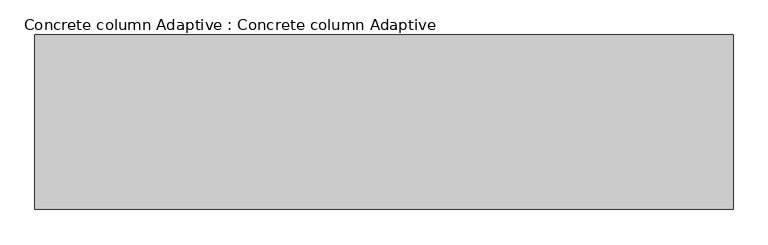
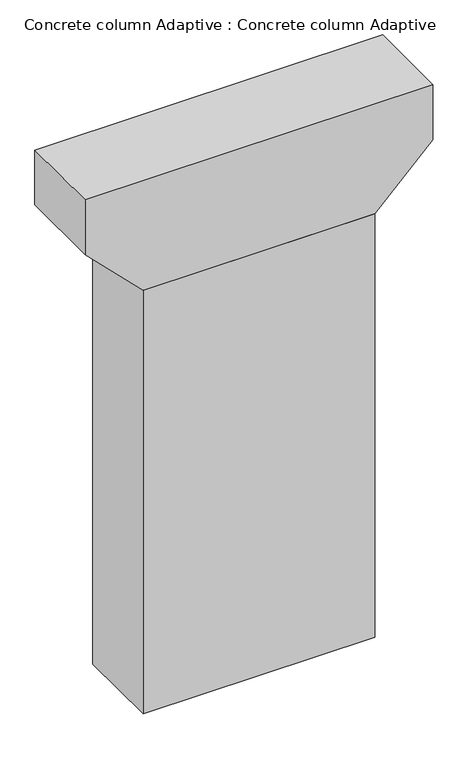
"""IFC4 building model written with IfcOpenShell, lengths in millimetres: proxy geometry, Concrete column Adaptive : Concrete column Adaptive."""

from ifc_helpers import new_model, si_unit, frame, origin, origin_with_axes, place, context, project, spatial, polyline, outline, extrude, source, transform, mapped, element, save


def concrete_column_adaptive_concrete_column_adaptive_030e40f1(model_context):
    return source(origin(), model_context, "Body", "SweptSolid", [
        extrude(outline(polyline([(19446.0, 6000.0), (19446.0, -6000.0), (17446.0, -6000.0), (15446.0, -4000.0), (15446.0, 4000.0), (17446.0, 6000.0), (19446.0, 6000.0)])), frame((0.0, -1500.0, 0.0), z_axis=(0.0, 1.0, 0.0), x_axis=(0.0, 0.0, 1.0)), (0.0, 0.0, 1.0), 3000.0),
        extrude(outline(polyline([(-4000.0, -1500.0), (-4000.0, 1500.0), (4000.0, 1500.0), (4000.0, -1500.0), (-4000.0, -1500.0)])), origin_with_axes(), (0.0, 0.0, 1.0), 15446.0),
    ])


if __name__ == "__main__":
    model = new_model("IFC4")
    model_context = context("Model", 3, world=origin())
    ifc_project = project(units=[si_unit("LENGTHUNIT", "METRE", prefix="MILLI")], contexts=[model_context])
    site = spatial("IfcSite", under=ifc_project)
    building = spatial("IfcBuilding", under=site)
    placement = place(None, origin())
    concrete_column_adaptive_concrete_column_adaptive_shape = concrete_column_adaptive_concrete_column_adaptive_030e40f1(model_context)
    element("IfcBuildingElementProxy", 1, Name="Concrete column Adaptive : Concrete column Adaptive", ObjectType="Concrete column Adaptive : Concrete column Adaptive", at=placement, inside=building, context=model_context, shape_type="MappedRepresentation", body=[
        mapped(concrete_column_adaptive_concrete_column_adaptive_shape, transform((0.0, 0.0, 0.0), x_axis=(1.0, 0.0, 0.0), y_axis=(0.0, 1.0, 0.0), z_axis=(0.0, 0.0, 1.0))),
    ])
    save(model, "model.ifc")

# Revit data of these elements
# Project information
#   Project Issue Date = "Issue Date"
#   Project Status = "Project Status"
#   Client Name = "Owner"
#   Project Address = "Enter address here"
#   Project Name = "Project Name"
#   Project Number = "Project Number"
# Type "Concrete column Adaptive : Concrete column Adaptive"
#   Height [instance default] = 30000 mm
#   Default Elevation = 0
# Element 1 (IfcBuildingElementProxy, "Concrete column Adaptive : Concrete column Adaptive")
#   Height = 15446 mm
